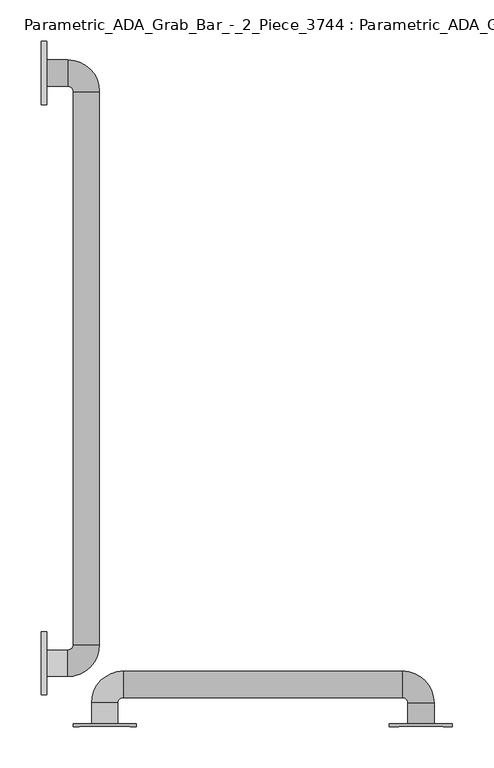
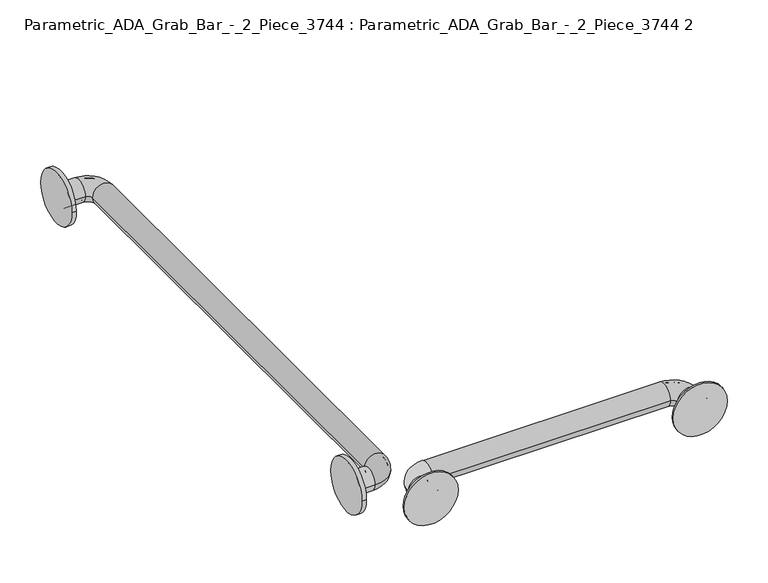
"""IFC4 building model written with IfcOpenShell, lengths in millimetres: proxy geometry, Parametric_ADA_Grab_Bar_-_2_Piece_3744 : Parametric_ADA_Grab_Bar_-_2_Piece_3744 2."""

from ifc_helpers import new_model, si_unit, point, frame, frame_2d, origin, place, context, project, spatial, polyline, circle_curve, ellipse_curve, trimmed, segment, composite_curve, outline, extrude, source, transform, mapped, element, save
from ifc_brep_helpers import plane_surface, cylinder_surface, revolved_surface, advanced_brep


def parametric_ada_grab_bar_2_piece_3744_parametric_ada_grab_bar_28af31cd(model_context):
    return source(origin(), model_context, "Body", "SolidModel", [
        advanced_brep(
        [(6.35, 884.2375, 838.2), (6.35, 915.9875, 838.2), (6.35, 887.4125, 838.2), (6.35, 912.8125, 838.2), (31.75, 884.2375, 838.2), (31.75, 915.9875, 838.2), (31.75, 887.4125, 838.2), (31.75, 912.8125, 838.2), (69.85, 877.8875, 838.2), (38.1, 877.8875, 838.2), (66.675, 877.8875, 838.2), (41.275, 877.8875, 838.2), (38.1, 211.1375, 838.2), (69.85, 211.1375, 838.2), (41.275, 211.1375, 838.2), (66.675, 211.1375, 838.2), (31.75, 173.0375, 838.2), (31.75, 204.7875, 838.2), (31.75, 176.2125, 838.2), (31.75, 201.6125, 838.2), (6.35, 204.7875, 838.2), (6.35, 173.0375, 838.2), (6.35, 201.6125, 838.2), (6.35, 176.2125, 838.2)],
        [
            (0, 1, circle_curve(frame((6.35, 900.1125, 838.2), z_axis=(-1.0, 0.0, 0.0), x_axis=(0.0, 1.0, 0.0)), 15.875)),
            (1, 0, circle_curve(frame((6.35, 900.1125, 838.2), z_axis=(-1.0, 0.0, 0.0), x_axis=(0.0, 1.0, 0.0)), 15.875)),
            (2, 3, circle_curve(frame((6.35, 900.1125, 838.2), z_axis=(1.0, 0.0, 0.0), x_axis=(0.0, 1.0, 0.0)), 12.7)),
            (3, 2, circle_curve(frame((6.35, 900.1125, 838.2), z_axis=(1.0, 0.0, 0.0), x_axis=(0.0, 1.0, 0.0)), 12.7)),
            (0, 4),
            (4, 5, circle_curve(frame((31.75, 900.1125, 838.2), z_axis=(-1.0, 0.0, 0.0), x_axis=(0.0, 1.0, 0.0)), 15.875)),
            (5, 1),
            (5, 4, circle_curve(frame((31.75, 900.1125, 838.2), z_axis=(-1.0, 0.0, 0.0), x_axis=(0.0, 1.0, 0.0)), 15.875)),
            (2, 6),
            (6, 7, circle_curve(frame((31.75, 900.1125, 838.2), z_axis=(1.0, 0.0, 0.0), x_axis=(0.0, 1.0, 0.0)), 12.7)),
            (7, 3),
            (7, 6, circle_curve(frame((31.75, 900.1125, 838.2), z_axis=(1.0, 0.0, 0.0), x_axis=(0.0, 1.0, 0.0)), 12.7)),
            (8, 5, circle_curve(frame((31.75, 877.8875, 838.2), z_axis=(0.0, 0.0, 1.0), x_axis=(0.0, 1.0, 0.0)), 38.1)),
            (4, 9, circle_curve(frame((31.75, 877.8875, 838.2), z_axis=(0.0, 0.0, -1.0), x_axis=(0.0, 1.0, 0.0)), 6.35)),
            (9, 8, circle_curve(frame((53.975, 877.8875, 838.2), z_axis=(0.0, 1.0, 0.0), x_axis=(1.0, 0.0, 0.0)), 15.875)),
            (8, 9, circle_curve(frame((53.975, 877.8875, 838.2), z_axis=(0.0, 1.0, 0.0), x_axis=(1.0, 0.0, 0.0)), 15.875)),
            (10, 7, circle_curve(frame((31.75, 877.8875, 838.2), z_axis=(0.0, 0.0, 1.0), x_axis=(0.0, 1.0, 0.0)), 34.925)),
            (6, 11, circle_curve(frame((31.75, 877.8875, 838.2), z_axis=(0.0, 0.0, -1.0), x_axis=(0.0, 1.0, 0.0)), 9.525)),
            (11, 10, circle_curve(frame((53.975, 877.8875, 838.2), z_axis=(0.0, -1.0, 0.0), x_axis=(1.0, 0.0, 0.0)), 12.7)),
            (10, 11, circle_curve(frame((53.975, 877.8875, 838.2), z_axis=(0.0, -1.0, 0.0), x_axis=(1.0, 0.0, 0.0)), 12.7)),
            (9, 12),
            (12, 13, circle_curve(frame((53.975, 211.1375, 838.2), z_axis=(0.0, 1.0, 0.0), x_axis=(1.0, 0.0, 0.0)), 15.875)),
            (13, 8),
            (13, 12, circle_curve(frame((53.975, 211.1375, 838.2), z_axis=(0.0, 1.0, 0.0), x_axis=(1.0, 0.0, 0.0)), 15.875)),
            (11, 14),
            (14, 15, circle_curve(frame((53.975, 211.1375, 838.2), z_axis=(0.0, -1.0, 0.0), x_axis=(1.0, 0.0, 0.0)), 12.7)),
            (15, 10),
            (15, 14, circle_curve(frame((53.975, 211.1375, 838.2), z_axis=(0.0, -1.0, 0.0), x_axis=(1.0, 0.0, 0.0)), 12.7)),
            (16, 13, circle_curve(frame((31.75, 211.1375, 838.2), z_axis=(0.0, 0.0, 1.0), x_axis=(1.0, 0.0, 0.0)), 38.1)),
            (12, 17, circle_curve(frame((31.75, 211.1375, 838.2), z_axis=(0.0, 0.0, -1.0), x_axis=(1.0, 0.0, 0.0)), 6.35)),
            (17, 16, circle_curve(frame((31.75, 188.9125, 838.2), z_axis=(1.0, -1.0770542613964651e-12, 0.0), x_axis=(-1.0770542613964651e-12, -1.0, 0.0)), 15.875)),
            (16, 17, circle_curve(frame((31.75, 188.9125, 838.2), z_axis=(1.0, 0.0, 0.0), x_axis=(0.0, -1.0, 0.0)), 15.875)),
            (18, 15, circle_curve(frame((31.75, 211.1375, 838.2), z_axis=(0.0, 0.0, 1.0), x_axis=(1.0, 0.0, 0.0)), 34.925)),
            (14, 19, circle_curve(frame((31.75, 211.1375, 838.2), z_axis=(0.0, 0.0, -1.0), x_axis=(1.0, 0.0, 0.0)), 9.525)),
            (19, 18, circle_curve(frame((31.75, 188.9125, 838.2), z_axis=(-1.0, 0.0, 0.0), x_axis=(0.0, -1.0, 0.0)), 12.7)),
            (18, 19, circle_curve(frame((31.75, 188.9125, 838.2), z_axis=(-1.0, 0.0, 0.0), x_axis=(0.0, -1.0, 0.0)), 12.7)),
            (20, 21, circle_curve(frame((6.35, 188.9125, 838.2), z_axis=(-1.0, 0.0, 0.0), x_axis=(0.0, -1.0, 0.0)), 15.875)),
            (21, 20, circle_curve(frame((6.35, 188.9125, 838.2), z_axis=(-1.0, 0.0, 0.0), x_axis=(0.0, -1.0, 0.0)), 15.875)),
            (22, 23, circle_curve(frame((6.35, 188.9125, 838.2), z_axis=(1.0, 0.0, 0.0), x_axis=(0.0, -1.0, 0.0)), 12.7)),
            (23, 22, circle_curve(frame((6.35, 188.9125, 838.2), z_axis=(1.0, 0.0, 0.0), x_axis=(0.0, -1.0, 0.0)), 12.7)),
            (17, 20),
            (21, 16),
            (19, 22),
            (23, 18),
        ],
        [
            plane_surface(frame((6.35, 900.1125, 838.2), z_axis=(-1.0, 0.0, 0.0), x_axis=(0.0, 0.0, 1.0))),
            cylinder_surface(frame((6.35, 900.1125, 838.2), z_axis=(-1.0, 0.0, 0.0), x_axis=(0.0, 1.0, 0.0)), 15.875),
            revolved_surface(polyline([(31.75, 912.8125, 838.2), (6.35, 912.8125, 838.2)]), (6.35, 900.1125, 838.2), (1.0, 0.0, 0.0)),
            revolved_surface(trimmed(ellipse_curve(frame((31.75, 900.1125, 838.2), z_axis=(-1.0, 0.0, 0.0), x_axis=(0.0, 1.0, 0.0)), 15.875, 15.875), [point((31.75, 884.2375, 838.2))], [point((31.75, 915.9875, 838.2))], True, "CARTESIAN"), (31.75, 877.8875, 838.2), (0.0, 0.0, -1.0)),
            revolved_surface(trimmed(ellipse_curve(frame((31.75, 900.1125, 838.2), z_axis=(-1.0, 0.0, 0.0), x_axis=(0.0, 1.0, 0.0)), 15.875, 15.875), [point((31.75, 915.9875, 838.2))], [point((31.75, 884.2375, 838.2))], True, "CARTESIAN"), (31.75, 877.8875, 838.2), (0.0, 0.0, -1.0)),
            revolved_surface(trimmed(ellipse_curve(frame((31.75, 900.1125, 838.2), z_axis=(1.0, 0.0, 0.0), x_axis=(0.0, 1.0, 0.0)), 12.7, 12.7), [point((31.75, 887.4125, 838.2))], [point((31.75, 912.8125, 838.2))], True, "CARTESIAN"), (31.75, 877.8875, 838.2), (0.0, 0.0, -1.0)),
            revolved_surface(trimmed(ellipse_curve(frame((31.75, 900.1125, 838.2), z_axis=(1.0, 0.0, 0.0), x_axis=(0.0, 1.0, 0.0)), 12.7, 12.7), [point((31.75, 912.8125, 838.2))], [point((31.75, 887.4125, 838.2))], True, "CARTESIAN"), (31.75, 877.8875, 838.2), (0.0, 0.0, -1.0)),
            cylinder_surface(frame((53.975, 877.8875, 838.2), z_axis=(0.0, 1.0, 0.0), x_axis=(1.0, 0.0, 0.0)), 15.875),
            revolved_surface(polyline([(66.675, 211.13750000000005, 838.2), (66.675, 877.8875, 838.2)]), (53.975, 877.8875, 838.2), (0.0, -1.0, 0.0)),
            revolved_surface(trimmed(ellipse_curve(frame((53.975, 211.1375, 838.2), z_axis=(0.0, 1.0, 0.0), x_axis=(1.0, 0.0, 0.0)), 15.875, 15.875), [point((38.1, 211.1375, 838.2))], [point((69.85, 211.1375, 838.2))], True, "CARTESIAN"), (31.75, 211.1375, 838.2), (0.0, 0.0, -1.0)),
            revolved_surface(trimmed(ellipse_curve(frame((53.975, 211.1375, 838.2), z_axis=(0.0, 1.0, 0.0), x_axis=(1.0, 0.0, 0.0)), 15.875, 15.875), [point((69.85, 211.1375, 838.2))], [point((38.1, 211.1375, 838.2))], True, "CARTESIAN"), (31.75, 211.1375, 838.2), (0.0, 0.0, -1.0)),
            revolved_surface(trimmed(ellipse_curve(frame((53.975, 211.1375, 838.2), z_axis=(0.0, -1.0, 0.0), x_axis=(1.0, 0.0, 0.0)), 12.7, 12.7), [point((41.275, 211.1375, 838.2))], [point((66.675, 211.1375, 838.2))], True, "CARTESIAN"), (31.75, 211.1375, 838.2), (0.0, 0.0, -1.0)),
            revolved_surface(trimmed(ellipse_curve(frame((53.975, 211.1375, 838.2), z_axis=(0.0, -1.0, 0.0), x_axis=(1.0, 0.0, 0.0)), 12.7, 12.7), [point((66.675, 211.1375, 838.2))], [point((41.275, 211.1375, 838.2))], True, "CARTESIAN"), (31.75, 211.1375, 838.2), (0.0, 0.0, -1.0)),
            plane_surface(frame((6.35, 188.9125, 838.2), z_axis=(-1.0, 0.0, 0.0), x_axis=(0.0, 0.0, 1.0))),
            cylinder_surface(frame((31.75, 188.9125, 838.2), z_axis=(1.0, 0.0, 0.0), x_axis=(0.0, -1.0, 0.0)), 15.875),
            revolved_surface(polyline([(6.350000000000001, 176.2125, 838.2), (31.75, 176.2125, 838.2)]), (31.75, 188.9125, 838.2), (-1.0, 0.0, 0.0)),
        ],
        [
            (0, [[1, 2], [3, 4]]),
            (1, [[-1, 5, 6, 7]]),
            (1, [[-2, -7, 8, -5]]),
            (2, [[-3, 9, 10, 11]]),
            (2, [[-4, -11, 12, -9]]),
            (3, [[13, -6, 14, 15]]),
            (4, [[-14, -8, -13, 16]]),
            (5, [[17, -10, 18, 19]]),
            (6, [[-18, -12, -17, 20]]),
            (7, [[-15, 21, 22, 23]]),
            (7, [[-16, -23, 24, -21]]),
            (8, [[-19, 25, 26, 27]]),
            (8, [[-20, -27, 28, -25]]),
            (9, [[29, -22, 30, 31]]),
            (10, [[-30, -24, -29, 32]]),
            (11, [[33, -26, 34, 35]]),
            (12, [[-34, -28, -33, 36]]),
            (13, [[37, 38], [39, 40]]),
            (14, [[-31, 41, -38, 42]]),
            (14, [[-32, -42, -37, -41]]),
            (15, [[-35, 43, -40, 44]]),
            (15, [[-36, -44, -39, -43]]),
        ],
    ),
        advanced_brep(
        [(92.075, 115.8875, 838.2), (60.325, 115.8875, 838.2), (88.9, 115.8875, 838.2), (63.5, 115.8875, 838.2), (92.075, 141.2875, 838.2), (60.325, 141.2875, 838.2), (88.9, 141.2875, 838.2), (63.5, 141.2875, 838.2), (98.425, 179.3875, 838.2), (98.425, 147.6375, 838.2), (98.425, 176.2125, 838.2), (98.425, 150.8125, 838.2), (434.975, 147.6375, 838.2), (434.975, 179.3875, 838.2), (434.975, 150.8125, 838.2), (434.975, 176.2125, 838.2), (473.075, 141.2875, 838.2), (441.325, 141.2875, 838.2), (469.9, 141.2875, 838.2), (444.5, 141.2875, 838.2), (441.325, 115.8875, 838.2), (473.075, 115.8875, 838.2), (444.5, 115.8875, 838.2), (469.9, 115.8875, 838.2)],
        [
            (0, 1, circle_curve(frame((76.2, 115.8875, 838.2), z_axis=(0.0, -1.0, 0.0), x_axis=(-1.0, 0.0, 0.0)), 15.875)),
            (1, 0, circle_curve(frame((76.2, 115.8875, 838.2), z_axis=(0.0, -1.0, 0.0), x_axis=(-1.0, 0.0, 0.0)), 15.875)),
            (2, 3, circle_curve(frame((76.2, 115.8875, 838.2), z_axis=(0.0, 1.0, 0.0), x_axis=(-1.0, 0.0, 0.0)), 12.7)),
            (3, 2, circle_curve(frame((76.2, 115.8875, 838.2), z_axis=(0.0, 1.0, 0.0), x_axis=(-1.0, 0.0, 0.0)), 12.7)),
            (0, 4),
            (4, 5, circle_curve(frame((76.2, 141.2875, 838.2), z_axis=(0.0, -1.0, 0.0), x_axis=(-1.0, 0.0, 0.0)), 15.875)),
            (5, 1),
            (5, 4, circle_curve(frame((76.2, 141.2875, 838.2), z_axis=(0.0, -1.0, 0.0), x_axis=(-1.0, 0.0, 0.0)), 15.875)),
            (2, 6),
            (6, 7, circle_curve(frame((76.2, 141.2875, 838.2), z_axis=(0.0, 1.0, 0.0), x_axis=(-1.0, 0.0, 0.0)), 12.7)),
            (7, 3),
            (7, 6, circle_curve(frame((76.2, 141.2875, 838.2), z_axis=(0.0, 1.0, 0.0), x_axis=(-1.0, 0.0, 0.0)), 12.7)),
            (8, 5, circle_curve(frame((98.425, 141.2875, 838.2), z_axis=(0.0, 0.0, 1.0), x_axis=(-1.0, 0.0, 0.0)), 38.1)),
            (4, 9, circle_curve(frame((98.425, 141.2875, 838.2), z_axis=(0.0, 0.0, -1.0), x_axis=(-1.0, 0.0, 0.0)), 6.35)),
            (9, 8, circle_curve(frame((98.425, 163.5125, 838.2), z_axis=(-1.0, 0.0, 0.0), x_axis=(0.0, 1.0, 0.0)), 15.875)),
            (8, 9, circle_curve(frame((98.425, 163.5125, 838.2), z_axis=(-1.0, 0.0, 0.0), x_axis=(0.0, 1.0, 0.0)), 15.875)),
            (10, 7, circle_curve(frame((98.425, 141.2875, 838.2), z_axis=(0.0, 0.0, 1.0), x_axis=(-1.0, 0.0, 0.0)), 34.925)),
            (6, 11, circle_curve(frame((98.425, 141.2875, 838.2), z_axis=(0.0, 0.0, -1.0), x_axis=(-1.0, 0.0, 0.0)), 9.525)),
            (11, 10, circle_curve(frame((98.425, 163.5125, 838.2), z_axis=(1.0, 0.0, 0.0), x_axis=(0.0, 1.0, 0.0)), 12.7)),
            (10, 11, circle_curve(frame((98.425, 163.5125, 838.2), z_axis=(1.0, 0.0, 0.0), x_axis=(0.0, 1.0, 0.0)), 12.7)),
            (9, 12),
            (12, 13, circle_curve(frame((434.975, 163.5125, 838.2), z_axis=(-1.0, 0.0, 0.0), x_axis=(0.0, 1.0, 0.0)), 15.875)),
            (13, 8),
            (13, 12, circle_curve(frame((434.975, 163.5125, 838.2), z_axis=(-1.0, 0.0, 0.0), x_axis=(0.0, 1.0, 0.0)), 15.875)),
            (11, 14),
            (14, 15, circle_curve(frame((434.975, 163.5125, 838.2), z_axis=(1.0, 0.0, 0.0), x_axis=(0.0, 1.0, 0.0)), 12.7)),
            (15, 10),
            (15, 14, circle_curve(frame((434.975, 163.5125, 838.2), z_axis=(1.0, 0.0, 0.0), x_axis=(0.0, 1.0, 0.0)), 12.7)),
            (16, 13, circle_curve(frame((434.975, 141.2875, 838.2), z_axis=(0.0, 0.0, 1.0), x_axis=(0.0, 1.0, 0.0)), 38.1)),
            (12, 17, circle_curve(frame((434.975, 141.2875, 838.2), z_axis=(0.0, 0.0, -1.0), x_axis=(0.0, 1.0, 0.0)), 6.35)),
            (17, 16, circle_curve(frame((457.2, 141.2875, 838.2), z_axis=(0.0, 1.0, 0.0), x_axis=(1.0, 0.0, 0.0)), 15.875)),
            (16, 17, circle_curve(frame((457.2, 141.2875, 838.2), z_axis=(0.0, 1.0, 0.0), x_axis=(1.0, 0.0, 0.0)), 15.875)),
            (18, 15, circle_curve(frame((434.975, 141.2875, 838.2), z_axis=(0.0, 0.0, 1.0), x_axis=(0.0, 1.0, 0.0)), 34.925)),
            (14, 19, circle_curve(frame((434.975, 141.2875, 838.2), z_axis=(0.0, 0.0, -1.0), x_axis=(0.0, 1.0, 0.0)), 9.525)),
            (19, 18, circle_curve(frame((457.2, 141.2875, 838.2), z_axis=(0.0, -1.0, 0.0), x_axis=(1.0, 0.0, 0.0)), 12.7)),
            (18, 19, circle_curve(frame((457.2, 141.2875, 838.2), z_axis=(0.0, -1.0, 0.0), x_axis=(1.0, 0.0, 0.0)), 12.7)),
            (20, 21, circle_curve(frame((457.2, 115.8875, 838.2), z_axis=(0.0, -1.0, 0.0), x_axis=(1.0, 0.0, 0.0)), 15.875)),
            (21, 20, circle_curve(frame((457.2, 115.8875, 838.2), z_axis=(0.0, -1.0, 0.0), x_axis=(1.0, 0.0, 0.0)), 15.875)),
            (22, 23, circle_curve(frame((457.2, 115.8875, 838.2), z_axis=(0.0, 1.0, 0.0), x_axis=(1.0, 0.0, 0.0)), 12.7)),
            (23, 22, circle_curve(frame((457.2, 115.8875, 838.2), z_axis=(0.0, 1.0, 0.0), x_axis=(1.0, 0.0, 0.0)), 12.7)),
            (17, 20),
            (21, 16),
            (19, 22),
            (23, 18),
        ],
        [
            plane_surface(frame((76.2, 115.8875, 838.2), z_axis=(0.0, -1.0, 0.0), x_axis=(0.0, 0.0, 1.0))),
            cylinder_surface(frame((76.2, 115.8875, 838.2), z_axis=(0.0, -1.0, 0.0), x_axis=(-1.0, 0.0, 0.0)), 15.875),
            revolved_surface(polyline([(63.5, 141.2875, 838.2), (63.5, 115.8875, 838.2)]), (76.2, 115.8875, 838.2), (0.0, 1.0, 0.0)),
            revolved_surface(trimmed(ellipse_curve(frame((76.2, 141.2875, 838.2), z_axis=(0.0, -1.0, 0.0), x_axis=(-1.0, 0.0, 0.0)), 15.875, 15.875), [point((92.075, 141.2875, 838.2))], [point((60.325, 141.2875, 838.2))], True, "CARTESIAN"), (98.425, 141.2875, 838.2), (0.0, 0.0, -1.0)),
            revolved_surface(trimmed(ellipse_curve(frame((76.2, 141.2875, 838.2), z_axis=(0.0, -1.0, 0.0), x_axis=(-1.0, 0.0, 0.0)), 15.875, 15.875), [point((60.325, 141.2875, 838.2))], [point((92.075, 141.2875, 838.2))], True, "CARTESIAN"), (98.425, 141.2875, 838.2), (0.0, 0.0, -1.0)),
            revolved_surface(trimmed(ellipse_curve(frame((76.2, 141.2875, 838.2), z_axis=(0.0, 1.0, 0.0), x_axis=(-1.0, 0.0, 0.0)), 12.7, 12.7), [point((88.9, 141.2875, 838.2))], [point((63.5, 141.2875, 838.2))], True, "CARTESIAN"), (98.425, 141.2875, 838.2), (0.0, 0.0, -1.0)),
            revolved_surface(trimmed(ellipse_curve(frame((76.2, 141.2875, 838.2), z_axis=(0.0, 1.0, 0.0), x_axis=(-1.0, 0.0, 0.0)), 12.7, 12.7), [point((63.5, 141.2875, 838.2))], [point((88.9, 141.2875, 838.2))], True, "CARTESIAN"), (98.425, 141.2875, 838.2), (0.0, 0.0, -1.0)),
            cylinder_surface(frame((98.425, 163.5125, 838.2), z_axis=(-1.0, 0.0, 0.0), x_axis=(0.0, 1.0, 0.0)), 15.875),
            revolved_surface(polyline([(434.975, 176.21249999999998, 838.2), (98.425, 176.21249999999998, 838.2)]), (98.425, 163.5125, 838.2), (1.0, 0.0, 0.0)),
            revolved_surface(trimmed(ellipse_curve(frame((434.975, 163.5125, 838.2), z_axis=(-1.0, 0.0, 0.0), x_axis=(0.0, 1.0, 0.0)), 15.875, 15.875), [point((434.975, 147.6375, 838.2))], [point((434.975, 179.3875, 838.2))], True, "CARTESIAN"), (434.975, 141.2875, 838.2), (0.0, 0.0, -1.0)),
            revolved_surface(trimmed(ellipse_curve(frame((434.975, 163.5125, 838.2), z_axis=(-1.0, 0.0, 0.0), x_axis=(0.0, 1.0, 0.0)), 15.875, 15.875), [point((434.975, 179.3875, 838.2))], [point((434.975, 147.6375, 838.2))], True, "CARTESIAN"), (434.975, 141.2875, 838.2), (0.0, 0.0, -1.0)),
            revolved_surface(trimmed(ellipse_curve(frame((434.975, 163.5125, 838.2), z_axis=(1.0, 0.0, 0.0), x_axis=(0.0, 1.0, 0.0)), 12.7, 12.7), [point((434.975, 150.8125, 838.2))], [point((434.975, 176.2125, 838.2))], True, "CARTESIAN"), (434.975, 141.2875, 838.2), (0.0, 0.0, -1.0)),
            revolved_surface(trimmed(ellipse_curve(frame((434.975, 163.5125, 838.2), z_axis=(1.0, 0.0, 0.0), x_axis=(0.0, 1.0, 0.0)), 12.7, 12.7), [point((434.975, 176.2125, 838.2))], [point((434.975, 150.8125, 838.2))], True, "CARTESIAN"), (434.975, 141.2875, 838.2), (0.0, 0.0, -1.0)),
            plane_surface(frame((457.2, 115.8875, 838.2), z_axis=(0.0, -1.0, 0.0), x_axis=(0.0, 0.0, 1.0))),
            cylinder_surface(frame((457.2, 141.2875, 838.2), z_axis=(0.0, 1.0, 0.0), x_axis=(1.0, 0.0, 0.0)), 15.875),
            revolved_surface(polyline([(469.9, 115.8875, 838.2), (469.9, 141.2875, 838.2)]), (457.2, 141.2875, 838.2), (0.0, -1.0, 0.0)),
        ],
        [
            (0, [[1, 2], [3, 4]]),
            (1, [[-1, 5, 6, 7]]),
            (1, [[-2, -7, 8, -5]]),
            (2, [[-3, 9, 10, 11]]),
            (2, [[-4, -11, 12, -9]]),
            (3, [[13, -6, 14, 15]]),
            (4, [[-14, -8, -13, 16]]),
            (5, [[17, -10, 18, 19]]),
            (6, [[-18, -12, -17, 20]]),
            (7, [[-15, 21, 22, 23]]),
            (7, [[-16, -23, 24, -21]]),
            (8, [[-19, 25, 26, 27]]),
            (8, [[-20, -27, 28, -25]]),
            (9, [[29, -22, 30, 31]]),
            (10, [[-30, -24, -29, 32]]),
            (11, [[33, -26, 34, 35]]),
            (12, [[-34, -28, -33, 36]]),
            (13, [[37, 38], [39, 40]]),
            (14, [[-31, 41, -38, 42]]),
            (14, [[-32, -42, -37, -41]]),
            (15, [[-35, 43, -40, 44]]),
            (15, [[-36, -44, -39, -43]]),
        ],
    ),
        extrude(outline(composite_curve([segment(trimmed(circle_curve(frame_2d((188.9125, 838.2)), 38.1), [point((150.8125, 838.2))], [point((227.0125, 838.2))], False, "CARTESIAN"), True, "CONTINUOUS"), segment(trimmed(circle_curve(frame_2d((188.9125, 838.2)), 38.1), [point((227.0125, 838.2))], [point((150.8125, 838.2))], False, "CARTESIAN"), True, "CONTINUOUS")], self_intersect=False)), frame((0.0, 0.0, 0.0), z_axis=(1.0, 0.0, 0.0), x_axis=(0.0, 1.0, 0.0)), (0.0, 0.0, 1.0), 6.35),
        extrude(outline(composite_curve([segment(trimmed(circle_curve(frame_2d((900.1125, 838.2)), 38.1), [point((862.0125, 838.2))], [point((938.2125, 838.2))], False, "CARTESIAN"), True, "CONTINUOUS"), segment(trimmed(circle_curve(frame_2d((900.1125, 838.2)), 38.1), [point((938.2125, 838.2))], [point((862.0125, 838.2))], False, "CARTESIAN"), True, "CONTINUOUS")], self_intersect=False)), frame((0.0, 0.0, 0.0), z_axis=(1.0, 0.0, 0.0), x_axis=(0.0, 1.0, 0.0)), (0.0, 0.0, 1.0), 6.35),
        extrude(outline(composite_curve([segment(trimmed(circle_curve(frame_2d((838.2, 457.2)), 38.1), [point((838.2, 495.3))], [point((838.2, 419.1))], False, "CARTESIAN"), True, "CONTINUOUS"), segment(trimmed(circle_curve(frame_2d((838.2, 457.2)), 38.1), [point((838.2, 419.1))], [point((838.2, 495.3))], False, "CARTESIAN"), True, "CONTINUOUS")], self_intersect=False)), frame((0.0, 112.7125, 0.0), z_axis=(0.0, 1.0, 0.0), x_axis=(0.0, 0.0, 1.0)), (0.0, 0.0, 1.0), 3.175),
        extrude(outline(composite_curve([segment(trimmed(circle_curve(frame_2d((838.2, 76.2)), 38.1), [point((838.2, 114.3))], [point((838.2, 38.1))], False, "CARTESIAN"), True, "CONTINUOUS"), segment(trimmed(circle_curve(frame_2d((838.2, 76.2)), 38.1), [point((838.2, 38.1))], [point((838.2, 114.3))], False, "CARTESIAN"), True, "CONTINUOUS")], self_intersect=False)), frame((0.0, 112.7125, 0.0), z_axis=(0.0, 1.0, 0.0), x_axis=(0.0, 0.0, 1.0)), (0.0, 0.0, 1.0), 3.175),
    ])


if __name__ == "__main__":
    model = new_model("IFC4")
    model_context = context("Model", 3, world=origin())
    ifc_project = project(units=[si_unit("LENGTHUNIT", "METRE", prefix="MILLI")], contexts=[model_context])
    site = spatial("IfcSite", under=ifc_project)
    building = spatial("IfcBuilding", under=site)
    placement = place(None, origin())
    parametric_ada_grab_bar_2_piece_3744_parametric_ada_grab_bar_shape = parametric_ada_grab_bar_2_piece_3744_parametric_ada_grab_bar_28af31cd(model_context)
    element("IfcBuildingElementProxy", 1, Name="Parametric_ADA_Grab_Bar_-_2_Piece_3744 : Parametric_ADA_Grab_Bar_-_2_Piece_3744 2", ObjectType="Parametric_ADA_Grab_Bar_-_2_Piece_3744 : Parametric_ADA_Grab_Bar_-_2_Piece_3744 2", at=placement, inside=building, context=model_context, shape_type="MappedRepresentation", body=[
        mapped(parametric_ada_grab_bar_2_piece_3744_parametric_ada_grab_bar_shape, transform((0.0, 0.0, 0.0), x_axis=(1.0, 0.0, 0.0), y_axis=(0.0, 1.0, 0.0), z_axis=(0.0, 0.0, 1.0))),
    ])
    save(model, "model.ifc")

# Revit data of these elements
# Type "Parametric_ADA_Grab_Bar_-_2_Piece_3744 : Parametric_ADA_Grab_Bar_-_2_Piece_3744 2"
#   Keynote = "M10281313.01"
#   Keynote = "M10281313.01"
#   offset from wall = 0' - 0 5/8"
#   Grab bar length (42" min) = 2' - 4"
#   Grab bar height = 2' - 9"
#   Grab bar Length (36" min) = 1' - 3"
#   Face of Wall to Grab bar (6" max) = 0' - 3"
#   Face of Wall to Grab bar (12" max) = 0' - 3"
# Element 1 (IfcBuildingElementProxy, "Parametric_ADA_Grab_Bar_-_2_Piece_3744 : Parametric_ADA_Grab_Bar_-_2_Piece_3744 2")
#   Materials on its faces: "Stainless Steel"
# Materials
#   "Stainless Steel": class "Metal", colour RGB 189 187 185, transparency 0, Description = "Stainless Steel 18/8", Cost = 0
